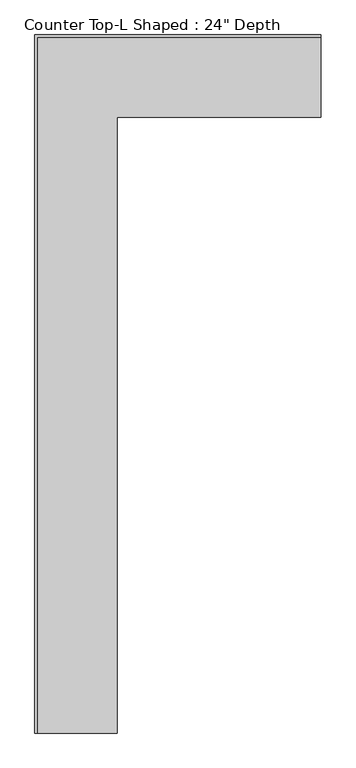
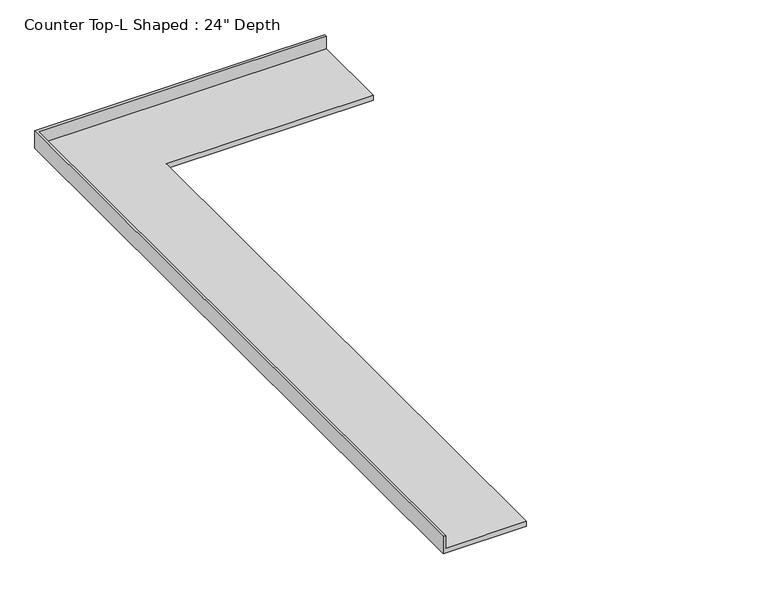
"""IFC4 building model written with IfcOpenShell, lengths in millimetres: furniture geometry."""

from ifc_helpers import new_model, si_unit, origin, place, context, project, spatial, faceted_brep, source, transform, mapped, element, save


def furniture_4175977f(model_context):
    return source(origin(), model_context, "Body", "Brep", [
        faceted_brep([(-565.4622951, -5384.8, 914.4), (-565.4622951, -635.0, 914.4), (1009.3377049, -635.0, 914.4), (1009.3377049, -19.05, 914.4), (-1181.4122951, -19.05, 914.4), (-1181.4122951, -5384.8, 914.4), (1009.3377049, 0.0, 876.3), (1009.3377049, -635.0, 876.3), (-565.4622951, -635.0, 876.3), (-565.4622951, -5384.8, 876.3), (-1200.4622951, -5384.8, 876.3), (-1200.4622951, 0.0, 876.3), (-1200.4622951, 0.0, 1016.0), (1009.3377049, 0.0, 1016.0), (-1200.4622951, -5384.8, 1016.0), (-1181.4122951, -5384.8, 1016.0), (1009.3377049, -19.05, 1016.0), (-1181.4122951, -19.05, 1016.0)], [[[0, 1, 2, 3, 4, 5]], [[6, 7, 8, 9, 10, 11]], [[6, 11, 12, 13]], [[11, 10, 14, 12]], [[14, 10, 9, 0, 5, 15]], [[1, 0, 9, 8]], [[2, 1, 8, 7]], [[7, 6, 13, 16, 3, 2]], [[12, 14, 15, 17, 16, 13]], [[3, 16, 17, 4]], [[17, 15, 5, 4]]]),
    ])


if __name__ == "__main__":
    model = new_model("IFC4")
    model_context = context("Model", 3, world=origin())
    ifc_project = project(units=[si_unit("LENGTHUNIT", "METRE", prefix="MILLI")], contexts=[model_context])
    site = spatial("IfcSite", under=ifc_project)
    building = spatial("IfcBuilding", under=site)
    placement = place(None, origin())
    furniture_shape = furniture_4175977f(model_context)
    element("IfcFurniture", 1, ObjectType="Counter Top-L Shaped : 24\" Depth", at=placement, inside=building, context=model_context, shape_type="MappedRepresentation", body=[
        mapped(furniture_shape, transform((0.0, 0.0, 0.0), x_axis=(1.0, 0.0, 0.0), y_axis=(0.0, 1.0, 0.0), z_axis=(0.0, 0.0, 1.0))),
    ])
    save(model, "model.ifc")

# Revit data of these elements
# Type "Counter Top-L Shaped : 24\" Depth"
#   Assembly Code = "C1030400"
#   Counter Thickness = 0' - 1 1/2"
#   Depth = 2' - 1"
#   Height = 3' - 0"
#   Length - Leg 1 [instance default] = 8' - 0"
#   Length - Leg 2 [instance default] = 6' - 0"
#   Counter Top Material = none
#   Default Elevation = 0
# Element 1 (IfcFurniture, "Counter Top-L Shaped : 24\" Depth")
#   Length - Leg 1 = 7' - 3"
#   Length - Leg 2 = 17' - 8"
#   Materials on its faces: "Counter Top"
# Materials
#   "Counter Top": class "Wood", colour RGB 226 177 128, transparency 0, Cost = 0
